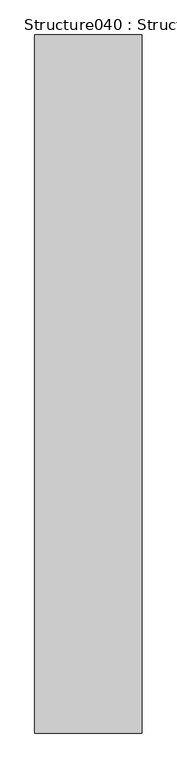
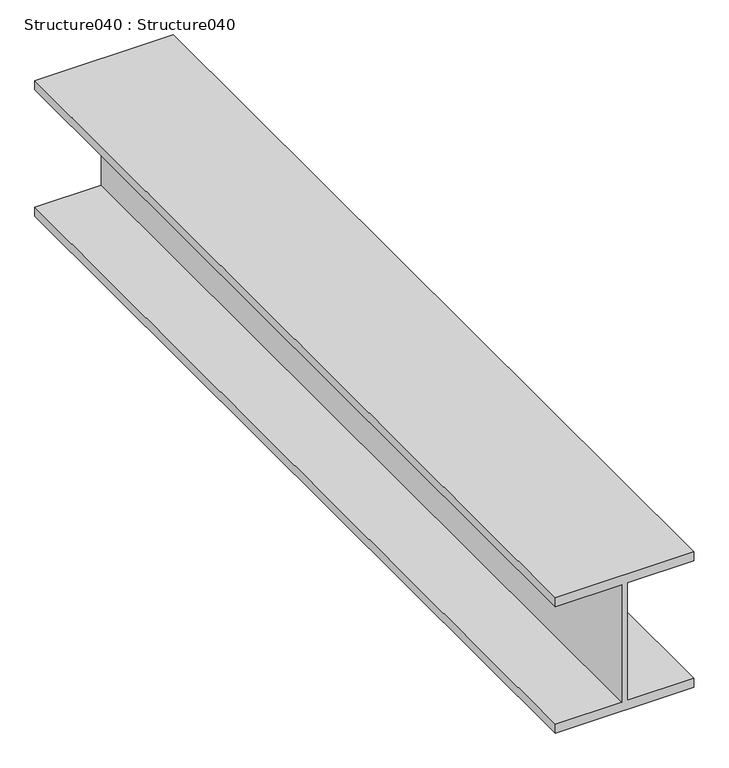
"""IFC4 building model written with IfcOpenShell, lengths in millimetres: proxy geometry, Structure040 : Structure040."""

import ifcopenshell
import ifcopenshell.guid

model = None  # the IFC model being written
_history = None  # IfcOwnerHistory: only IFC2X3 demands one
_inside = {}  # id of a spatial element -> (the spatial element, [elements in it])
_under = {}  # id of a project, library or spatial element -> (it, [spatial elements below it])
_declared = {}  # id of a project -> (the project, [libraries it declares])
_typed = {}  # id of a type object -> (the type object, [elements of that type])
_made_of = {}  # id of a material, layer set ... -> (it, [elements and type objects made of it])


def new_model(schema):
    """Start an empty IFC model of exactly this schema.

    Asked for "IFC4X3", IfcOpenShell would pick the latest addendum, in which some entities
    have other attributes; the version numbers below select the first issue.
    IFC2X3 requires an IfcOwnerHistory on every rooted entity: one is made here for all.
    """
    global model, _history
    if schema == "IFC4X3":
        model = ifcopenshell.file(schema_version=(4, 3, 0, 0))
    else:
        model = ifcopenshell.file(schema=schema)
    _inside.clear()
    _under.clear()
    _declared.clear()
    _typed.clear()
    _made_of.clear()
    _history = None
    if model.schema == "IFC2X3":
        org = make("IfcOrganization", Name="unknown")
        user = make(
            "IfcPersonAndOrganization",
            ThePerson=make("IfcPerson", FamilyName="unknown"),
            TheOrganization=org,
        )
        app = make(
            "IfcApplication",
            ApplicationDeveloper=org,
            Version="unknown",
            ApplicationFullName="unknown",
            ApplicationIdentifier="unknown",
        )
        _history = make(
            "IfcOwnerHistory",
            OwningUser=user,
            OwningApplication=app,
            ChangeAction="ADDED",
            CreationDate=0,
        )
    return model


def make(cls, **values):
    """One entity of the class cls with the attributes given. An attribute that is None is left unset."""
    return model.create_entity(
        cls, **{name: value for name, value in values.items() if value is not None}
    )


def rooted(cls, **values):
    """An entity with a GlobalId (a new one), such as an element, a storey or a relation."""
    return make(cls, GlobalId=ifcopenshell.guid.new(), OwnerHistory=_history, **values)


def si_unit(unit_type, name, prefix=None):
    """IfcSIUnit, for example si_unit("LENGTHUNIT", "METRE", prefix="MILLI")."""
    return make("IfcSIUnit", UnitType=unit_type, Prefix=prefix, Name=name)


def assignment(units):
    """IfcUnitAssignment: the units of a project."""
    return None if units is None else make("IfcUnitAssignment", Units=units)


def point(xyz):
    """IfcCartesianPoint."""
    return None if xyz is None else make("IfcCartesianPoint", Coordinates=xyz)


def direction(xyz):
    """IfcDirection."""
    return None if xyz is None else make("IfcDirection", DirectionRatios=xyz)


def frame(location, z_axis=None, x_axis=None):
    """IfcAxis2Placement3D, a coordinate frame: its origin and axes. An axis left out is left unset."""
    return make(
        "IfcAxis2Placement3D",
        Location=point(location),
        Axis=direction(z_axis),
        RefDirection=direction(x_axis),
    )


def origin():
    """The frame at (0, 0, 0) with its axes left unset."""
    return frame((0.0, 0.0, 0.0))


def place(relative_to, where):
    """IfcLocalPlacement: puts the frame where relative to a parent placement (None: the world)."""
    return make(
        "IfcLocalPlacement", PlacementRelTo=relative_to, RelativePlacement=where
    )


def context(
    kind, dimensions, precision=None, world=None, true_north=None, identifier=None
):
    """IfcGeometricRepresentationContext, for example the 3D "Model" context."""
    return make(
        "IfcGeometricRepresentationContext",
        ContextIdentifier=identifier,
        ContextType=kind,
        CoordinateSpaceDimension=dimensions,
        Precision=precision,
        WorldCoordinateSystem=world,
        TrueNorth=true_north,
    )


def project(units=None, contexts=None):
    """IfcProject with its units and contexts."""
    return rooted(
        "IfcProject",
        Name="project",
        RepresentationContexts=contexts,
        UnitsInContext=assignment(units),
    )


def spatial(cls, under=None, at=None, **own):
    """A site, building, storey or space (cls), placed at a placement, below another one or the project."""
    s = rooted(cls, ObjectPlacement=at, **own)
    if under is not None:
        _under.setdefault(under.id(), (under, []))[1].append(s)
    return s


def polyline(points):
    """IfcPolyline through the points."""
    return make("IfcPolyline", Points=[point(p) for p in points])


def outline(outer, holes=None, kind="AREA"):
    """IfcArbitraryClosedProfileDef: a profile drawn as a closed curve; with holes, ...WithVoids."""
    if holes is None:
        return make("IfcArbitraryClosedProfileDef", ProfileType=kind, OuterCurve=outer)
    return make(
        "IfcArbitraryProfileDefWithVoids",
        ProfileType=kind,
        OuterCurve=outer,
        InnerCurves=holes,
    )


def extrude(swept, where, along, depth):
    """IfcExtrudedAreaSolid: the profile swept, set in the frame where, extruded along a direction by depth."""
    return make(
        "IfcExtrudedAreaSolid",
        SweptArea=swept,
        Position=where,
        ExtrudedDirection=direction(along),
        Depth=depth,
    )


def shape(context_of_items, identifier, shape_type, items):
    """IfcShapeRepresentation: the items that make up one representation, for example the "Body"."""
    return make(
        "IfcShapeRepresentation",
        ContextOfItems=context_of_items,
        RepresentationIdentifier=identifier,
        RepresentationType=shape_type,
        Items=items,
    )


def source(mapping_origin, context_of_items, identifier, shape_type, items):
    """IfcRepresentationMap: a shape defined once, which mapped items show again and again."""
    return make(
        "IfcRepresentationMap",
        MappingOrigin=mapping_origin,
        MappedRepresentation=shape(context_of_items, identifier, shape_type, items),
    )


def transform(
    local_origin,
    x_axis=None,
    y_axis=None,
    z_axis=None,
    scale=None,
    scale2=None,
    scale3=None,
    uniform=True,
):
    """IfcCartesianTransformationOperator3D, or its non-uniform kind. x_axis, y_axis, z_axis: its Axis1, 2, 3."""
    if uniform:
        return make(
            "IfcCartesianTransformationOperator3D",
            Axis1=direction(x_axis),
            Axis2=direction(y_axis),
            LocalOrigin=point(local_origin),
            Scale=scale,
            Axis3=direction(z_axis),
        )
    return make(
        "IfcCartesianTransformationOperator3DnonUniform",
        Axis1=direction(x_axis),
        Axis2=direction(y_axis),
        LocalOrigin=point(local_origin),
        Scale=scale,
        Axis3=direction(z_axis),
        Scale2=scale2,
        Scale3=scale3,
    )


def mapped(mapping_source, mapping_target):
    """IfcMappedItem: shows the shape of a source again, moved by a transform."""
    return make(
        "IfcMappedItem", MappingSource=mapping_source, MappingTarget=mapping_target
    )


def made_of(thing, what):
    """Note that an element or type object is made of a material, layer set ...; save() writes the relation."""
    if what is not None:
        _made_of.setdefault(what.id(), (what, []))[1].append(thing)
    return thing


def element(
    cls,
    number,
    at=None,
    inside=None,
    cuts=None,
    type_object=None,
    material=None,
    context=None,
    identifier="Body",
    shape_type=None,
    held_by="IfcProductDefinitionShape",
    body=None,
    shapes=None,
    **own,
):
    """One element of the class cls, such as IfcWall. Its Tag is "e" and its number.

    at: its placement. inside: the storey or other place that contains it. cuts: it is an
    opening in that element (IfcRelVoidsElement). A single representation is given by context,
    identifier, shape_type and body (its items); several are given by shapes. held_by: the class
    of the entity that holds the representations. save() writes the other relations.
    """
    e = rooted(cls, Tag="e%d" % number, ObjectPlacement=at, **own)
    if body is not None:
        shapes = [shape(context, identifier, shape_type, body)]
    if shapes is not None:
        e.Representation = make(held_by, Representations=shapes)
    if inside is not None:
        _inside.setdefault(inside.id(), (inside, []))[1].append(e)
    if cuts is not None:
        rooted(
            "IfcRelVoidsElement", RelatingBuildingElement=cuts, RelatedOpeningElement=e
        )
    if type_object is not None:
        _typed.setdefault(type_object.id(), (type_object, []))[1].append(e)
    return made_of(e, material)


def aggregate(whole, parts):
    """IfcRelAggregates: a whole, such as a stair, and the parts it consists of."""
    return rooted("IfcRelAggregates", RelatingObject=whole, RelatedObjects=parts)


def save(model, path):
    """Write the relations noted so far, then the file.

    IfcRelAggregates (storeys below a building ...), IfcRelContainedInSpatialStructure (elements
    in a storey), IfcRelDefinesByType, IfcRelAssociatesMaterial and IfcRelDeclares: one each for
    every whole, place, type object, material and project.
    """
    for whole, parts in _under.values():
        aggregate(whole, parts)
    for where, things in _inside.values():
        rooted(
            "IfcRelContainedInSpatialStructure",
            RelatedElements=things,
            RelatingStructure=where,
        )
    for kind, things in _typed.values():
        rooted("IfcRelDefinesByType", RelatedObjects=things, RelatingType=kind)
    for what, things in _made_of.values():
        rooted("IfcRelAssociatesMaterial", RelatedObjects=things, RelatingMaterial=what)
    for by, libraries in _declared.values():
        rooted("IfcRelDeclares", RelatingContext=by, RelatedDefinitions=libraries)
    model.write(path)


def structure040_structure040_909150ff(model_context):
    return source(origin(), model_context, "Body", "SweptSolid", [
        extrude(outline(polyline([(40028.622, -4828.5743825), (39752.27, -4828.5743825), (39752.27, -4975.7038825), (39731.696, -4975.7038825), (39731.696, -4668.3638825), (39752.27, -4668.3638825), (39752.27, -4815.4933825), (40028.622, -4815.4933825), (40028.622, -4668.3638825), (40049.196, -4668.3638825), (40049.196, -4975.7038825), (40028.622, -4975.7038825), (40028.622, -4828.5743825)])), frame((0.0, -1052.8906574, 0.0), z_axis=(0.0, 1.0, 0.0), x_axis=(0.0, 0.0, 1.0)), (0.0, 0.0, 1.0), 2000.0),
    ])


if __name__ == "__main__":
    model = new_model("IFC4")
    model_context = context("Model", 3, world=origin())
    ifc_project = project(units=[si_unit("LENGTHUNIT", "METRE", prefix="MILLI")], contexts=[model_context])
    site = spatial("IfcSite", under=ifc_project)
    building = spatial("IfcBuilding", under=site)
    placement = place(None, origin())
    structure040_structure040_shape = structure040_structure040_909150ff(model_context)
    element("IfcBuildingElementProxy", 1, Name="Structure040 : Structure040", ObjectType="Structure040 : Structure040", at=placement, inside=building, context=model_context, shape_type="MappedRepresentation", body=[
        mapped(structure040_structure040_shape, transform((0.0, 0.0, 0.0), x_axis=(1.0, 0.0, 0.0), y_axis=(0.0, 1.0, 0.0), z_axis=(0.0, 0.0, 1.0))),
    ])
    save(model, "model.ifc")

# Revit data of these elements
# Type "Structure040 : Structure040"
#   NameOverride = "Structure040"
# Element 1 (IfcBuildingElementProxy, "Structure040 : Structure040")
#   Materials on its faces: "STEEL STRUCTURE (SEE STRUCTURAL DWGS)"
# Materials
#   "STEEL STRUCTURE (SEE STRUCTURAL DWGS)": class "Unassigned", colour RGB 128 128 128, transparency 0, Cost = 0
